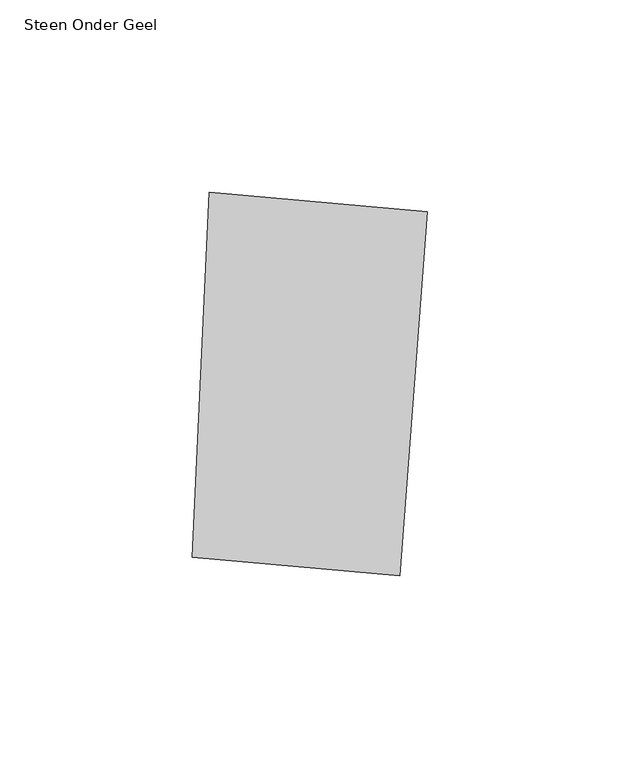
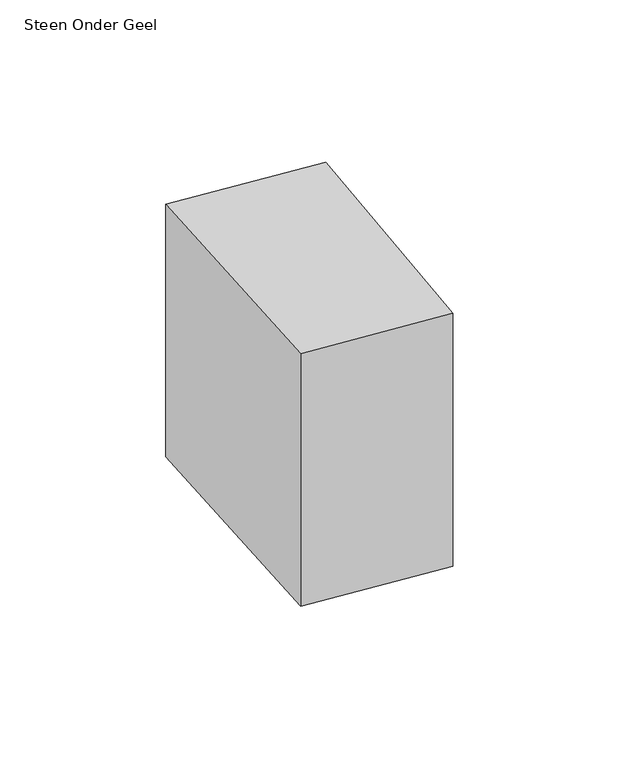
"""IFC4 building model written with IfcOpenShell, lengths in millimetres: proxy geometry, 00_GMA_steen_versie_4 : Steen Onder Geel."""

from ifc_helpers import new_model, si_unit, origin, origin_with_axes, place, context, project, spatial, polyline, outline, extrude, source, transform, mapped, element, save


def steen_onder_geel_64f296b9(model_context):
    return source(origin(), model_context, "Body", "SweptSolid", [
        extrude(outline(polyline([(103.9691139, 113.9237418), (96.8005202, 19.1835658), (42.7132909, 24.0720297), (47.1163594, 119.0658014), (103.9691139, 113.9237418)])), origin_with_axes(), (0.0, 0.0, 1.0), 100.0),
    ])


if __name__ == "__main__":
    model = new_model("IFC4")
    model_context = context("Model", 3, world=origin())
    ifc_project = project(units=[si_unit("LENGTHUNIT", "METRE", prefix="MILLI")], contexts=[model_context])
    site = spatial("IfcSite", under=ifc_project)
    building = spatial("IfcBuilding", under=site)
    placement = place(None, origin())
    steen_onder_geel_shape = steen_onder_geel_64f296b9(model_context)
    element("IfcBuildingElementProxy", 1, Name="00_GMA_steen_versie_4 : Steen Onder Geel", ObjectType="00_GMA_steen_versie_4 : Steen Onder Geel", at=placement, inside=building, context=model_context, shape_type="MappedRepresentation", body=[
        mapped(steen_onder_geel_shape, transform((0.0, 0.0, 0.0), x_axis=(1.0, 0.0, 0.0), y_axis=(0.0, 1.0, 0.0), z_axis=(0.0, 0.0, 1.0))),
    ])
    save(model, "model.ifc")

# Revit data of these elements
# Type "00_GMA_steen_versie_4 : Steen Onder Geel"
#   StootVoegHalfBoven [instance default] = 5 mm
#   StootVoegHalf [instance default] = 5 mm
#   StootVoegBreedteOnder = 10 mm
#   StootVoegBreedteBoven = 10 mm
#   Steendikte = 100 mm
#   LintVoegOnderHalf = 0 mm
#   LintVoegOnder = 0 mm
#   LintVoegBovenHalf = 5 mm
#   LintVoegBoven = 10 mm
#   materiaal = 21_steen_geel
#   MateriaalVoeg = none
#   Default Elevation = 0
# Element 1 (IfcBuildingElementProxy, "00_GMA_steen_versie_4 : Steen Onder Geel")
#   Materials on its faces: "21_steen_geel"
# Materials
#   "21_steen_geel": class "Unassigned", colour RGB 202 202 0, transparency 0, Cost = 0
